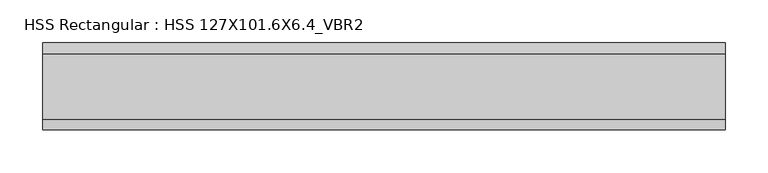
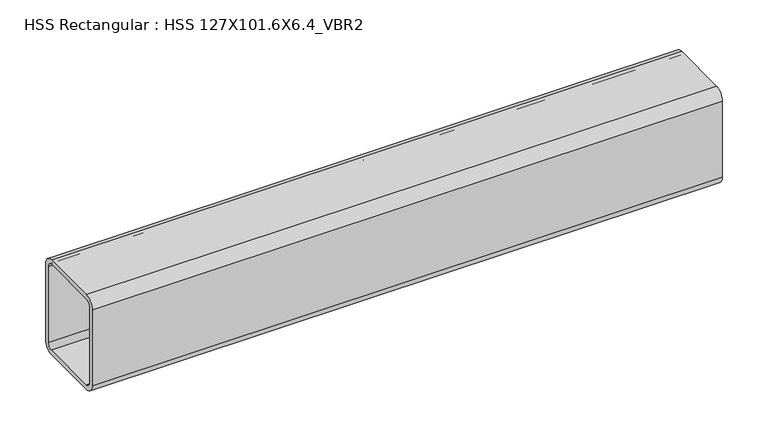
"""IFC4 building model written with IfcOpenShell, lengths in millimetres: member geometry, HSS Rectangular : HSS 127X101.6X6.4_VBR2."""

from ifc_helpers import new_model, si_unit, point, frame, frame_2d, origin, place, context, project, spatial, polyline, circle_curve, trimmed, segment, composite_curve, outline, extrude, source, transform, mapped, element, save


def hss_rectangular_hss_127x101_6x6_4_vbr2_6751103c(model_context):
    return source(origin(), model_context, "Body", "SweptSolid", [
        extrude(outline(composite_curve([segment(polyline([(50.8, 50.8), (50.8, -50.8)]), True, "CONTINUOUS"), segment(trimmed(circle_curve(frame_2d((38.1, -50.8)), 12.7), [point((50.8, -50.8))], [point((38.1, -63.5))], False, "CARTESIAN"), True, "CONTINUOUS"), segment(polyline([(38.1, -63.5), (-38.1, -63.5)]), True, "CONTINUOUS"), segment(trimmed(circle_curve(frame_2d((-38.1, -50.8)), 12.7), [point((-38.1, -63.5))], [point((-50.8, -50.8))], False, "CARTESIAN"), True, "CONTINUOUS"), segment(polyline([(-50.8, -50.8), (-50.8, 50.8)]), True, "CONTINUOUS"), segment(trimmed(circle_curve(frame_2d((-38.1, 50.8)), 12.7), [point((-50.8, 50.8))], [point((-38.1, 63.5))], False, "CARTESIAN"), True, "CONTINUOUS"), segment(polyline([(-38.1, 63.5), (38.1, 63.5)]), True, "CONTINUOUS"), segment(trimmed(circle_curve(frame_2d((38.1, 50.8)), 12.7), [point((38.1, 63.5))], [point((50.8, 50.8))], False, "CARTESIAN"), True, "CONTINUOUS")], self_intersect=False), holes=[composite_curve([segment(trimmed(circle_curve(frame_2d((-38.1, 50.8)), 6.35), [point((-38.1, 57.15))], [point((-44.45, 50.8))], True, "CARTESIAN"), True, "CONTINUOUS"), segment(polyline([(-44.45, 50.8), (-44.45, -50.8)]), True, "CONTINUOUS"), segment(trimmed(circle_curve(frame_2d((-38.1, -50.8)), 6.35), [point((-44.45, -50.8))], [point((-38.1, -57.15))], True, "CARTESIAN"), True, "CONTINUOUS"), segment(polyline([(-38.1, -57.15), (38.1, -57.15)]), True, "CONTINUOUS"), segment(trimmed(circle_curve(frame_2d((38.1, -50.8)), 6.35), [point((38.1, -57.15))], [point((44.45, -50.8))], True, "CARTESIAN"), True, "CONTINUOUS"), segment(polyline([(44.45, -50.8), (44.45, 50.8)]), True, "CONTINUOUS"), segment(trimmed(circle_curve(frame_2d((38.1, 50.8)), 6.35), [point((44.45, 50.8))], [point((38.1, 57.15))], True, "CARTESIAN"), True, "CONTINUOUS"), segment(polyline([(38.1, 57.15), (-38.1, 57.15)]), True, "CONTINUOUS")], self_intersect=False)]), frame((-414.7902003, 0.0, 0.0), z_axis=(1.0, 0.0, 0.0), x_axis=(0.0, 1.0, 0.0)), (0.0, 0.0, 1.0), 795.9948039),
    ])


if __name__ == "__main__":
    model = new_model("IFC4")
    model_context = context("Model", 3, world=origin())
    ifc_project = project(units=[si_unit("LENGTHUNIT", "METRE", prefix="MILLI")], contexts=[model_context])
    site = spatial("IfcSite", under=ifc_project)
    building = spatial("IfcBuilding", under=site)
    placement = place(None, origin())
    hss_rectangular_hss_127x101_6x6_4_vbr2_shape = hss_rectangular_hss_127x101_6x6_4_vbr2_6751103c(model_context)
    element("IfcMember", 1, ObjectType="HSS Rectangular : HSS 127X101.6X6.4_VBR2", at=placement, inside=building, context=model_context, shape_type="MappedRepresentation", body=[
        mapped(hss_rectangular_hss_127x101_6x6_4_vbr2_shape, transform((0.0, 0.0, 0.0), x_axis=(1.0, 0.0, 0.0), y_axis=(0.0, 1.0, 0.0), z_axis=(0.0, 0.0, 1.0))),
    ])
    save(model, "model.ifc")

# Revit data of these elements
# Type "HSS Rectangular : HSS 127X101.6X6.4_VBR2"
#   Section Name Key = "HSS5X4X1/4"
#   Assembly Code = "B10"
#   Width = 10.16 cm
#   Wall Nominal Thickness = 0.635 cm
#   Wall Design Thickness = 0.5918 cm
#   Torsional Moment of Inertia = 749.217 cm⁴
#   Torsional Modulus = 136.34 cm³
#   Section Area = 24.7741 cm²
#   Plastic Modulus weak axis = 91.2759 cm³
#   Plastic Modulus strong axis = 106.352 cm³
#   Perimeter = 0.435254 m²/m
#   Outer Fillet = 1.27 cm
#   Nominal Weight = 20.7004 kgf/m
#   Moment of Inertia weak axis = 393.755 cm⁴
#   Moment of Inertia strong axis = 557.75 cm⁴
#   Inner Fillet = 0.635 cm
#   Height = 12.7 cm
#   Elastic Modulus weak axis = 77.5108 cm³
#   Elastic Modulus strong axis = 87.6708 cm³
#   Centroid Vertical = 6.35 cm
#   Centroid Horizontal = 5.08 cm
#   Length [instance default] = 1524 mm
#   Structural Material [instance default] = Steel ASTM A500, Grade C, Rectangular and Square
#   Principal Axes Angle = 0
# Element 1 (IfcMember, "HSS Rectangular : HSS 127X101.6X6.4_VBR2")
#   Materials on its faces: "Steel ASTM A500, Grade C, Rectangular and Square"
# Materials
#   "Steel ASTM A500, Grade C, Rectangular and Square": class "Metal", colour RGB 120 120 120, transparency 0, Description = "Carbon steel", Cost = 0
